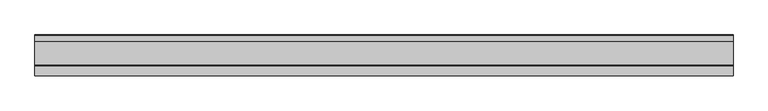
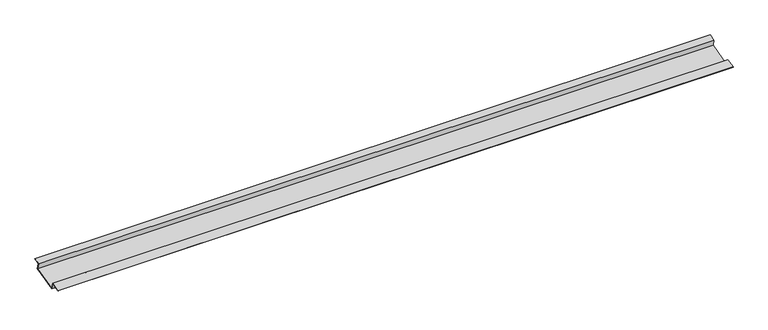
"""IFC4 building model written with IfcOpenShell, lengths in millimetres: proxy geometry, Soffit005 3553 : Soffit005 3553."""

from ifc_helpers import new_model, si_unit, frame, origin, place, context, project, spatial, polyline, outline, extrude, source, transform, mapped, element, save


def generic_models_08c13545(model_context):
    return source(origin(), model_context, "Body", "SweptSolid", [
        extrude(outline(polyline([(10667.4844028, 43464.7253726), (10672.1227691, 43446.2082609), (10598.2064546, 43427.6929037), (10593.5680888, 43446.2151657), (10568.0989149, 43439.8371464), (10567.7904064, 43441.0691052), (10594.4915391, 43447.7556331), (10599.1298846, 43429.2334518), (10670.5822412, 43447.1316102), (10665.9438547, 43465.6488027), (10684.5002367, 43470.2957128), (10684.8087452, 43469.063754), (10667.4844028, 43464.7253726)])), frame((3694.0383192, 0.0, 0.0), z_axis=(1.0, 0.0, 0.0), x_axis=(0.0, 1.0, 0.0)), (0.0, 0.0, 1.0), 2000.25),
    ])


if __name__ == "__main__":
    model = new_model("IFC4")
    model_context = context("Model", 3, world=origin())
    ifc_project = project(units=[si_unit("LENGTHUNIT", "METRE", prefix="MILLI")], contexts=[model_context])
    site = spatial("IfcSite", under=ifc_project)
    building = spatial("IfcBuilding", under=site)
    placement = place(None, origin())
    generic_models_shape = generic_models_08c13545(model_context)
    element("IfcBuildingElementProxy", 1, Name="Soffit005 3553 : Soffit005 3553", ObjectType="Soffit005 3553 : Soffit005 3553", at=placement, inside=building, context=model_context, shape_type="MappedRepresentation", body=[
        mapped(generic_models_shape, transform((0.0, 0.0, 0.0), x_axis=(1.0, 0.0, 0.0), y_axis=(0.0, 1.0, 0.0), z_axis=(0.0, 0.0, 1.0))),
    ])
    save(model, "model.ifc")

# Revit data of these elements
# Type "Soffit005 3553 : Soffit005 3553"
#   NameOverride = "Soffit005"
# Element 1 (IfcBuildingElementProxy, "Soffit005 3553 : Soffit005 3553")
#   Materials on its faces: "16 GA. COPPER SOFFIT VENT - VERIFY W/ ARCHITECT ON LOCATION"
# Materials
#   "16 GA. COPPER SOFFIT VENT - VERIFY W/ ARCHITECT ON LOCATION": class "Unassigned", colour RGB 85 255 127, transparency 0
